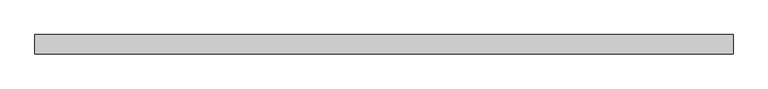
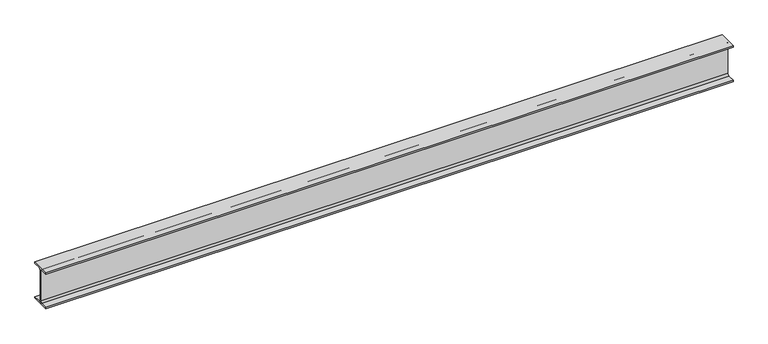
"""IFC4 building model written with IfcOpenShell, lengths in millimetres: beam geometry, 0912_Steel Framing_H-KSD3502 : H_SB_ASB_H-250x125x6x9."""

from ifc_helpers import new_model, si_unit, point, frame, frame_2d, origin, place, context, project, spatial, polyline, circle_curve, trimmed, segment, composite_curve, outline, extrude, source, transform, mapped, element, save


def beam_c25b449d(model_context):
    return source(origin(), model_context, "Body", "SweptSolid", [
        extrude(outline(composite_curve([segment(polyline([(62.5, -116.0), (62.5, -125.0), (-62.5, -125.0), (-62.5, -116.0), (-15.0, -116.0)]), True, "CONTINUOUS"), segment(trimmed(circle_curve(frame_2d((-15.0, -104.0)), 12.0), [point((-15.0, -116.0))], [point((-3.0, -104.0))], True, "CARTESIAN"), True, "CONTINUOUS"), segment(polyline([(-3.0, -104.0), (-3.0, 104.0)]), True, "CONTINUOUS"), segment(trimmed(circle_curve(frame_2d((-15.0, 104.0)), 12.0), [point((-3.0, 104.0))], [point((-15.0, 116.0))], True, "CARTESIAN"), True, "CONTINUOUS"), segment(polyline([(-15.0, 116.0), (-62.5, 116.0), (-62.5, 125.0), (62.5, 125.0), (62.5, 116.0), (15.0, 116.0)]), True, "CONTINUOUS"), segment(trimmed(circle_curve(frame_2d((15.0, 104.0)), 12.0), [point((15.0, 116.0))], [point((3.0, 104.0))], True, "CARTESIAN"), True, "CONTINUOUS"), segment(polyline([(3.0, 104.0), (3.0, -104.0)]), True, "CONTINUOUS"), segment(trimmed(circle_curve(frame_2d((15.0, -104.0)), 12.0), [point((3.0, -104.0))], [point((15.0, -116.0))], True, "CARTESIAN"), True, "CONTINUOUS"), segment(polyline([(15.0, -116.0), (62.5, -116.0)]), True, "CONTINUOUS")], self_intersect=False)), frame((-2164.4729123, 0.0, 0.0), z_axis=(1.0, 0.0, 0.0), x_axis=(0.0, 1.0, 0.0)), (0.0, 0.0, 1.0), 4526.7729123),
    ])


if __name__ == "__main__":
    model = new_model("IFC4")
    model_context = context("Model", 3, world=origin())
    ifc_project = project(units=[si_unit("LENGTHUNIT", "METRE", prefix="MILLI")], contexts=[model_context])
    site = spatial("IfcSite", under=ifc_project)
    building = spatial("IfcBuilding", under=site)
    placement = place(None, origin())
    beam_shape = beam_c25b449d(model_context)
    element("IfcBeam", 1, ObjectType="0912_Steel Framing_H-KSD3502 : H_SB_ASB_H-250x125x6x9", at=placement, inside=building, context=model_context, shape_type="MappedRepresentation", body=[
        mapped(beam_shape, transform((0.0, 0.0, 0.0), x_axis=(1.0, 0.0, 0.0), y_axis=(0.0, 1.0, 0.0), z_axis=(0.0, 0.0, 1.0))),
    ])
    save(model, "model.ifc")

# Revit data of these elements
# Type "0912_Steel Framing_H-KSD3502 : H_SB_ASB_H-250x125x6x9"
#   H_WM Code_1 = "S01AA003-00001 | Main Steel Structure Fabrication Work | Shelter/Building | Light Steel - Standard (30KG/M>Weight) | Material: (   )"
#   H_WM Code_2 = "S03AA029-00001 | Main Steel Structure Erection Work | Shelter/Building | Light Steel (30KG/M>Weight) | Material: (   )"
#   H_WM Code_3 = "S01AA010-00001 | Main Steel Structure Fabrication Work | Shelter/Building | Steel Painting/Coating | for Non-Fireproofed Steel Surface, Surface Preparation, Primer, Second & Final Coat | Material: (   )"
#   H_Q'ty Cal Type Tag = "SB-Q2"
#   Width = 12.5 cm
#   Web Thickness = 0.6 cm
#   Web Fillet = 1.2 cm
#   Warping Constant = 42539.8 cm⁶
#   W = 0
#   Torsional Moment of Inertia = 7.8102 cm⁴
#   Section Area = 37.66 cm²
#   Plastic Modulus weak axis = 73.1 cm³
#   Plastic Modulus strong axis = 366.0 cm³
#   Perimeter = 0.97 m²/m
#   Nominal Weight = 29.60 kgf/m
#   Moment of Inertia weak axis = 294.00 cm⁴
#   Moment of Inertia strong axis = 4050.00 cm⁴
#   Height = 25.0 cm
#   Flange Thickness = 0.9 cm
#   Elastic Modulus weak axis = 47.0 cm³
#   Elastic Modulus strong axis = 324.0 cm³
#   Centroid Vertical = 12.5 cm
#   Centroid Horizontal = 6.25 cm
#   Ix = 40500000
#   Length [instance default] = 1.5240 m
#   Zx = 366000
#   b = 0.1250 m
#   h = 0.2500 m
#   r = 0.0120 m
#   s = 0.0060 m
#   t = 0.0090 m
#   A = 0.003766 m²
#   Structural Material [instance default] = Steel, 45-345
#   Assembly Code = ""
# Element 1 (IfcBeam, "0912_Steel Framing_H-KSD3502 : H_SB_ASB_H-250x125x6x9")
#   Structural Material = none
# Materials
#   "Steel, 45-345": class "Metal", colour RGB 189 187 185, transparency 0, Description = "Steel 345 MPa", Cost = 0
